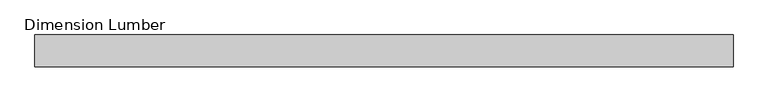
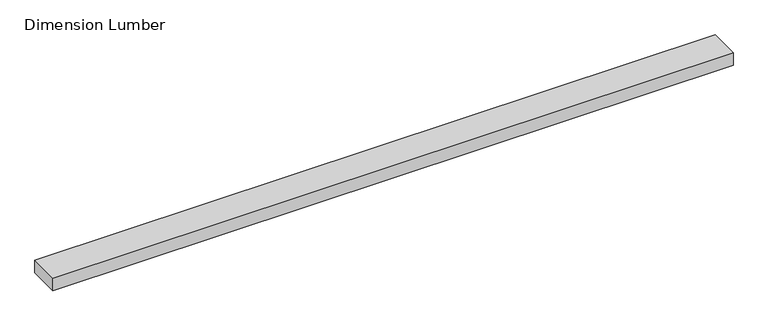
"""IFC4 building model written with IfcOpenShell, lengths in millimetres: beam geometry, Dimension Lumber : Top Supporting Lumbers."""

import ifcopenshell
import ifcopenshell.guid

model = None  # the IFC model being written
_history = None  # IfcOwnerHistory: only IFC2X3 demands one
_inside = {}  # id of a spatial element -> (the spatial element, [elements in it])
_under = {}  # id of a project, library or spatial element -> (it, [spatial elements below it])
_declared = {}  # id of a project -> (the project, [libraries it declares])
_typed = {}  # id of a type object -> (the type object, [elements of that type])
_made_of = {}  # id of a material, layer set ... -> (it, [elements and type objects made of it])


def new_model(schema):
    """Start an empty IFC model of exactly this schema.

    Asked for "IFC4X3", IfcOpenShell would pick the latest addendum, in which some entities
    have other attributes; the version numbers below select the first issue.
    IFC2X3 requires an IfcOwnerHistory on every rooted entity: one is made here for all.
    """
    global model, _history
    if schema == "IFC4X3":
        model = ifcopenshell.file(schema_version=(4, 3, 0, 0))
    else:
        model = ifcopenshell.file(schema=schema)
    _inside.clear()
    _under.clear()
    _declared.clear()
    _typed.clear()
    _made_of.clear()
    _history = None
    if model.schema == "IFC2X3":
        org = make("IfcOrganization", Name="unknown")
        user = make(
            "IfcPersonAndOrganization",
            ThePerson=make("IfcPerson", FamilyName="unknown"),
            TheOrganization=org,
        )
        app = make(
            "IfcApplication",
            ApplicationDeveloper=org,
            Version="unknown",
            ApplicationFullName="unknown",
            ApplicationIdentifier="unknown",
        )
        _history = make(
            "IfcOwnerHistory",
            OwningUser=user,
            OwningApplication=app,
            ChangeAction="ADDED",
            CreationDate=0,
        )
    return model


def make(cls, **values):
    """One entity of the class cls with the attributes given. An attribute that is None is left unset."""
    return model.create_entity(
        cls, **{name: value for name, value in values.items() if value is not None}
    )


def rooted(cls, **values):
    """An entity with a GlobalId (a new one), such as an element, a storey or a relation."""
    return make(cls, GlobalId=ifcopenshell.guid.new(), OwnerHistory=_history, **values)


def si_unit(unit_type, name, prefix=None):
    """IfcSIUnit, for example si_unit("LENGTHUNIT", "METRE", prefix="MILLI")."""
    return make("IfcSIUnit", UnitType=unit_type, Prefix=prefix, Name=name)


def assignment(units):
    """IfcUnitAssignment: the units of a project."""
    return None if units is None else make("IfcUnitAssignment", Units=units)


def point(xyz):
    """IfcCartesianPoint."""
    return None if xyz is None else make("IfcCartesianPoint", Coordinates=xyz)


def direction(xyz):
    """IfcDirection."""
    return None if xyz is None else make("IfcDirection", DirectionRatios=xyz)


def frame(location, z_axis=None, x_axis=None):
    """IfcAxis2Placement3D, a coordinate frame: its origin and axes. An axis left out is left unset."""
    return make(
        "IfcAxis2Placement3D",
        Location=point(location),
        Axis=direction(z_axis),
        RefDirection=direction(x_axis),
    )


def origin():
    """The frame at (0, 0, 0) with its axes left unset."""
    return frame((0.0, 0.0, 0.0))


def place(relative_to, where):
    """IfcLocalPlacement: puts the frame where relative to a parent placement (None: the world)."""
    return make(
        "IfcLocalPlacement", PlacementRelTo=relative_to, RelativePlacement=where
    )


def context(
    kind, dimensions, precision=None, world=None, true_north=None, identifier=None
):
    """IfcGeometricRepresentationContext, for example the 3D "Model" context."""
    return make(
        "IfcGeometricRepresentationContext",
        ContextIdentifier=identifier,
        ContextType=kind,
        CoordinateSpaceDimension=dimensions,
        Precision=precision,
        WorldCoordinateSystem=world,
        TrueNorth=true_north,
    )


def project(units=None, contexts=None):
    """IfcProject with its units and contexts."""
    return rooted(
        "IfcProject",
        Name="project",
        RepresentationContexts=contexts,
        UnitsInContext=assignment(units),
    )


def spatial(cls, under=None, at=None, **own):
    """A site, building, storey or space (cls), placed at a placement, below another one or the project."""
    s = rooted(cls, ObjectPlacement=at, **own)
    if under is not None:
        _under.setdefault(under.id(), (under, []))[1].append(s)
    return s


def polyline(points):
    """IfcPolyline through the points."""
    return make("IfcPolyline", Points=[point(p) for p in points])


def outline(outer, holes=None, kind="AREA"):
    """IfcArbitraryClosedProfileDef: a profile drawn as a closed curve; with holes, ...WithVoids."""
    if holes is None:
        return make("IfcArbitraryClosedProfileDef", ProfileType=kind, OuterCurve=outer)
    return make(
        "IfcArbitraryProfileDefWithVoids",
        ProfileType=kind,
        OuterCurve=outer,
        InnerCurves=holes,
    )


def extrude(swept, where, along, depth):
    """IfcExtrudedAreaSolid: the profile swept, set in the frame where, extruded along a direction by depth."""
    return make(
        "IfcExtrudedAreaSolid",
        SweptArea=swept,
        Position=where,
        ExtrudedDirection=direction(along),
        Depth=depth,
    )


def shape(context_of_items, identifier, shape_type, items):
    """IfcShapeRepresentation: the items that make up one representation, for example the "Body"."""
    return make(
        "IfcShapeRepresentation",
        ContextOfItems=context_of_items,
        RepresentationIdentifier=identifier,
        RepresentationType=shape_type,
        Items=items,
    )


def source(mapping_origin, context_of_items, identifier, shape_type, items):
    """IfcRepresentationMap: a shape defined once, which mapped items show again and again."""
    return make(
        "IfcRepresentationMap",
        MappingOrigin=mapping_origin,
        MappedRepresentation=shape(context_of_items, identifier, shape_type, items),
    )


def transform(
    local_origin,
    x_axis=None,
    y_axis=None,
    z_axis=None,
    scale=None,
    scale2=None,
    scale3=None,
    uniform=True,
):
    """IfcCartesianTransformationOperator3D, or its non-uniform kind. x_axis, y_axis, z_axis: its Axis1, 2, 3."""
    if uniform:
        return make(
            "IfcCartesianTransformationOperator3D",
            Axis1=direction(x_axis),
            Axis2=direction(y_axis),
            LocalOrigin=point(local_origin),
            Scale=scale,
            Axis3=direction(z_axis),
        )
    return make(
        "IfcCartesianTransformationOperator3DnonUniform",
        Axis1=direction(x_axis),
        Axis2=direction(y_axis),
        LocalOrigin=point(local_origin),
        Scale=scale,
        Axis3=direction(z_axis),
        Scale2=scale2,
        Scale3=scale3,
    )


def mapped(mapping_source, mapping_target):
    """IfcMappedItem: shows the shape of a source again, moved by a transform."""
    return make(
        "IfcMappedItem", MappingSource=mapping_source, MappingTarget=mapping_target
    )


def made_of(thing, what):
    """Note that an element or type object is made of a material, layer set ...; save() writes the relation."""
    if what is not None:
        _made_of.setdefault(what.id(), (what, []))[1].append(thing)
    return thing


def element(
    cls,
    number,
    at=None,
    inside=None,
    cuts=None,
    type_object=None,
    material=None,
    context=None,
    identifier="Body",
    shape_type=None,
    held_by="IfcProductDefinitionShape",
    body=None,
    shapes=None,
    **own,
):
    """One element of the class cls, such as IfcWall. Its Tag is "e" and its number.

    at: its placement. inside: the storey or other place that contains it. cuts: it is an
    opening in that element (IfcRelVoidsElement). A single representation is given by context,
    identifier, shape_type and body (its items); several are given by shapes. held_by: the class
    of the entity that holds the representations. save() writes the other relations.
    """
    e = rooted(cls, Tag="e%d" % number, ObjectPlacement=at, **own)
    if body is not None:
        shapes = [shape(context, identifier, shape_type, body)]
    if shapes is not None:
        e.Representation = make(held_by, Representations=shapes)
    if inside is not None:
        _inside.setdefault(inside.id(), (inside, []))[1].append(e)
    if cuts is not None:
        rooted(
            "IfcRelVoidsElement", RelatingBuildingElement=cuts, RelatedOpeningElement=e
        )
    if type_object is not None:
        _typed.setdefault(type_object.id(), (type_object, []))[1].append(e)
    return made_of(e, material)


def aggregate(whole, parts):
    """IfcRelAggregates: a whole, such as a stair, and the parts it consists of."""
    return rooted("IfcRelAggregates", RelatingObject=whole, RelatedObjects=parts)


def save(model, path):
    """Write the relations noted so far, then the file.

    IfcRelAggregates (storeys below a building ...), IfcRelContainedInSpatialStructure (elements
    in a storey), IfcRelDefinesByType, IfcRelAssociatesMaterial and IfcRelDeclares: one each for
    every whole, place, type object, material and project.
    """
    for whole, parts in _under.values():
        aggregate(whole, parts)
    for where, things in _inside.values():
        rooted(
            "IfcRelContainedInSpatialStructure",
            RelatedElements=things,
            RelatingStructure=where,
        )
    for kind, things in _typed.values():
        rooted("IfcRelDefinesByType", RelatedObjects=things, RelatingType=kind)
    for what, things in _made_of.values():
        rooted("IfcRelAssociatesMaterial", RelatedObjects=things, RelatingMaterial=what)
    for by, libraries in _declared.values():
        rooted("IfcRelDeclares", RelatingContext=by, RelatedDefinitions=libraries)
    model.write(path)


def dimension_lumber_f00769ea(model_context):
    return source(origin(), model_context, "Body", "SweptSolid", [
        extrude(outline(polyline([(927.1, 44.45), (927.1, -44.45), (-1016.0, -44.45), (-1016.0, 44.45), (927.1, 44.45)])), frame((0.0, 0.0, -19.05), z_axis=(0.0, 0.0, 1.0), x_axis=(1.0, 0.0, 0.0)), (0.0, 0.0, 1.0), 38.1),
    ])


if __name__ == "__main__":
    model = new_model("IFC4")
    model_context = context("Model", 3, world=origin())
    ifc_project = project(units=[si_unit("LENGTHUNIT", "METRE", prefix="MILLI")], contexts=[model_context])
    site = spatial("IfcSite", under=ifc_project)
    building = spatial("IfcBuilding", under=site)
    placement = place(None, origin())
    dimension_lumber_shape = dimension_lumber_f00769ea(model_context)
    element("IfcBeam", 1, ObjectType="Dimension Lumber : Top Supporting Lumbers", at=placement, inside=building, context=model_context, shape_type="MappedRepresentation", body=[
        mapped(dimension_lumber_shape, transform((0.0, 0.0, 0.0), x_axis=(1.0, 0.0, 0.0), y_axis=(0.0, 1.0, 0.0), z_axis=(0.0, 0.0, 1.0))),
    ])
    save(model, "model.ifc")

# Revit data of these elements
# Type "Dimension Lumber : Top Supporting Lumbers"
#   Assembly Code = "B10"
#   A = 0.0364583 SF
#   Length [instance default] = 5' - 0"
#   b = 0' - 3 1/2"
#   d = 0' - 1 1/2"
#   Structural Material [instance default] = Softwood, Lumber
# Element 1 (IfcBeam, "Dimension Lumber : Top Supporting Lumbers")
#   Structural Material = Douglas Fir #2
#   Materials on its faces: "Douglas Fir #2"
# Materials
#   "Softwood, Lumber": class "Wood", colour RGB 223 192 134, transparency 0, Description = "Pinus Echinata", Cost = 0
#   "Douglas Fir #2": class "Wood", colour RGB 223 192 134, transparency 0, Description = "Pinus Echinata", Cost = 0
